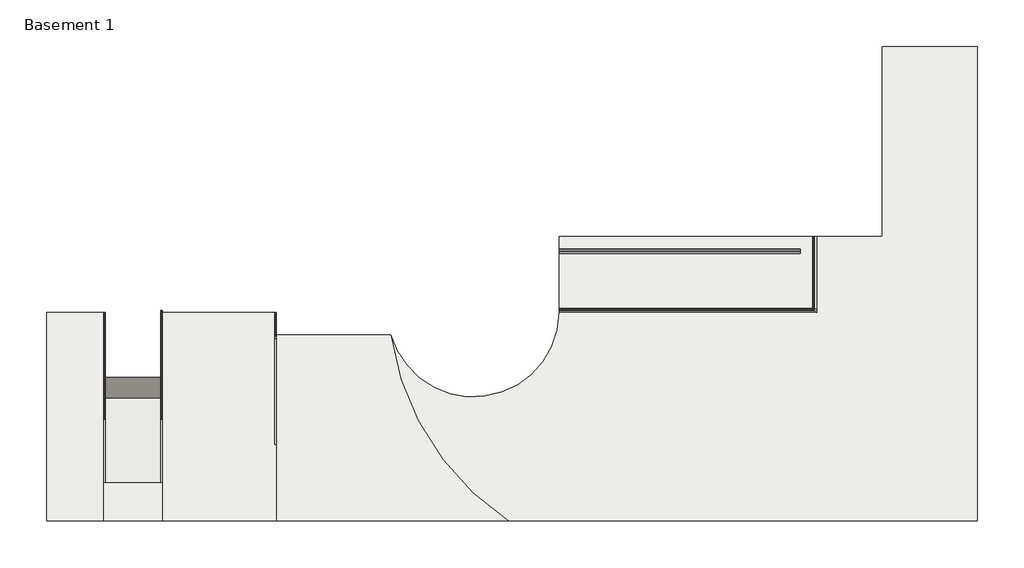
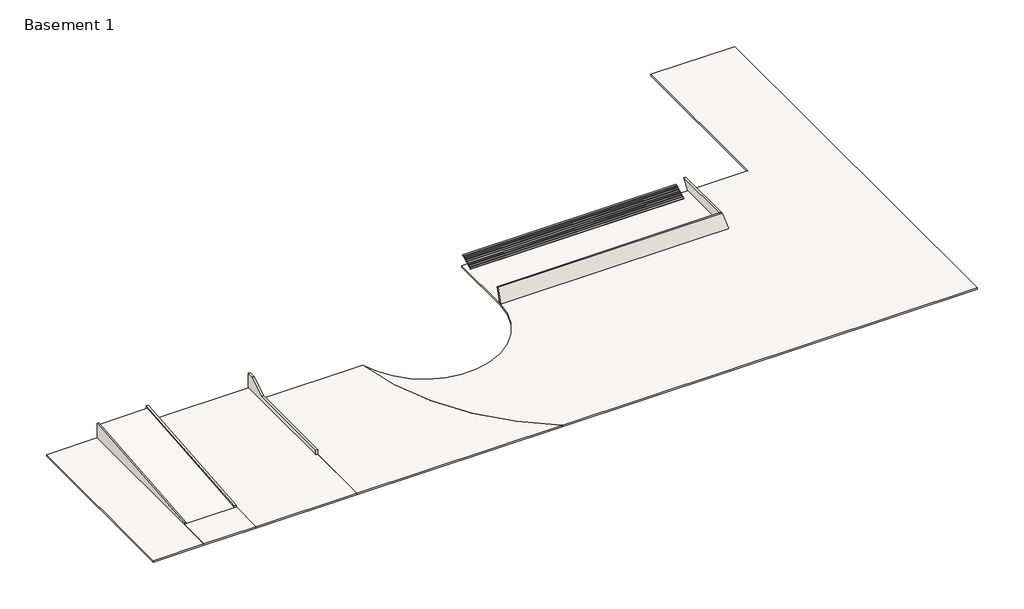
# One storey: 6 slabs, 5 walls, 1 stair flight.
"""IFC4 building model written with IfcOpenShell, lengths in millimetres."""

from ifc_helpers import new_model, si_unit, point, frame, frame_2d, origin, place, context, project, spatial, polyline, circle_curve, ellipse_curve, trimmed, segment, composite_curve, outline, extrude, faceted_brep, element, save
from ifc_brep_helpers import plane_surface, revolved_surface, advanced_brep

model = new_model("IFC4")

# Units and contexts
model_context = context("Model", 3, world=origin())
ifc_project = project(units=[si_unit("LENGTHUNIT", "METRE", prefix="MILLI")], contexts=[model_context])

# Site, building, storey
site = spatial("IfcSite", under=ifc_project)
building = spatial("IfcBuilding", under=site)
storey = spatial("IfcBuildingStorey", under=building, Name="Basement 1", Elevation=-2590.8)

# Slabs
placement = place(None, origin())
element("IfcSlab", 1, ObjectType="a_drive", at=placement, inside=storey, context=model_context, shape_type="SweptSolid", body=[
    extrude(outline(polyline([(19188.911889, -458.4117136), (-8130.1793721, -2896.8117136), (-8130.1793721, -2590.8), (19188.911889, -152.4), (19188.911889, -458.4117136)])), frame((-52722.4307976, 0.0, 0.0), z_axis=(1.0, 0.0, 0.0), x_axis=(0.0, 1.0, 0.0)), (0.0, 0.0, 1.0), 8839.2),
])
element("IfcSlab", 2, ObjectType="a_drive", at=placement, inside=storey, context=model_context, shape_type="SweptSolid", body=[
    extrude(outline(polyline([(-53027.2307976, -8130.1793721), (-43578.4307976, -8130.1793721), (-43578.4307976, -14339.088111), (-53027.2307976, -14339.088111), (-53027.2307976, -8130.1793721)])), frame((0.0, 0.0, -2895.6), z_axis=(0.0, 0.0, 1.0), x_axis=(1.0, 0.0, 0.0)), (0.0, 0.0, 1.0), 304.8),
])
element("IfcSlab", 3, ObjectType="a_site field", at=placement, inside=storey, context=model_context, shape_type="SweptSolid", body=[
    extrude(outline(composite_curve([segment(polyline([(20124.7692024, 31380.911889), (71940.7692024, 31380.911889), (71940.7692024, 61860.911889), (87180.7692024, 61860.911889), (87180.7692024, -14339.088111), (11898.6110424, -14339.088111)]), True, "CONTINUOUS"), segment(trimmed(circle_curve(frame_2d((35078.8556976, 21137.4265857)), 42378.1410317), [point((11898.6110424, -14339.088111))], [point((-6930.2202358, 15556.7118891))], False, "CARTESIAN"), True, "CONTINUOUS"), segment(trimmed(circle_curve(frame_2d((6325.7581451, 19397.6292514)), 13801.2176644), [point((-6930.2202358, 15556.7118891))], [point((20124.7692024, 19150.8442002))], True, "CARTESIAN"), True, "CONTINUOUS"), segment(polyline([(20124.7692024, 19150.8442002), (20124.7692024, 31380.911889)]), True, "CONTINUOUS")], self_intersect=False)), frame((0.0, 0.0, -2895.6), z_axis=(0.0, 0.0, 1.0), x_axis=(1.0, 0.0, 0.0)), (0.0, 0.0, 1.0), 304.8),
])
element("IfcSlab", 4, ObjectType="a_site field", at=placement, inside=storey, context=model_context, shape_type="SweptSolid", body=[
    extrude(outline(polyline([(-62171.2307976, 19188.911889), (-53027.2307976, 19188.911889), (-53027.2307976, -14339.088111), (-62171.2307976, -14339.088111), (-62171.2307976, 19188.911889)])), frame((0.0, 0.0, -2895.6), z_axis=(0.0, 0.0, 1.0), x_axis=(1.0, 0.0, 0.0)), (0.0, 0.0, 1.0), 304.8),
])
element("IfcSlab", 5, ObjectType="a_site field", at=placement, inside=storey, context=model_context, shape_type="SweptSolid", body=[
    extrude(outline(polyline([(-43578.4307976, 19188.911889), (-25290.4307976, 19188.911889), (-25290.4307976, -14339.088111), (-43578.4307976, -14339.088111), (-43578.4307976, 19188.911889)])), frame((0.0, 0.0, -2895.6), z_axis=(0.0, 0.0, 1.0), x_axis=(1.0, 0.0, 0.0)), (0.0, 0.0, 1.0), 304.8),
])
element("IfcSlab", 6, ObjectType="a_site paving", at=placement, inside=storey, context=model_context, shape_type="SweptSolid", body=[
    extrude(outline(composite_curve([segment(polyline([(-25290.4307976, 15556.711889), (-6930.2202358, 15556.711889)]), True, "CONTINUOUS"), segment(trimmed(circle_curve(frame_2d((35907.4785274, 21659.3058951)), 43270.1986236), [point((-6930.2202358, 15556.711889))], [point((11898.6110424, -14339.088111))], True, "CARTESIAN"), True, "CONTINUOUS"), segment(polyline([(11898.6110424, -14339.088111), (-25290.4307976, -14339.088111), (-25290.4307976, 15556.711889)]), True, "CONTINUOUS")], self_intersect=False)), frame((0.0, 0.0, -2895.6), z_axis=(0.0, 0.0, 1.0), x_axis=(1.0, 0.0, 0.0)), (0.0, 0.0, 1.0), 304.8),
])

# Stair flight
element("IfcStairFlight", 7, ObjectType="3/4\" Nosing", at=placement, inside=storey, context=model_context, shape_type="Brep", body=[
    faceted_brep([(58732.7692024, 28637.711889, -1507.0666667), (20124.7692024, 28637.711889, -1507.0666667), (20124.7692024, 28656.761889, -1676.4), (58732.7692024, 28656.761889, -1676.4), (58732.7692024, 28961.561889, -1507.0666667), (20124.7692024, 28961.561889, -1507.0666667), (20124.7692024, 28961.561889, -1579.7080571), (20124.7692024, 28787.5163918, -1676.4), (58732.7692024, 28787.5163918, -1676.4), (58732.7692024, 28961.561889, -1579.7080571), (20124.7692024, 28942.511889, -1337.7333333), (58732.7692024, 28942.511889, -1337.7333333), (58732.7692024, 29266.361889, -1337.7333333), (20124.7692024, 29266.361889, -1337.7333333), (20124.7692024, 29266.361889, -1410.3747238), (58732.7692024, 29266.361889, -1410.3747238), (20124.7692024, 29571.161889, -1241.0413904), (20124.7692024, 29875.961889, -1071.7080571), (20124.7692024, 30180.761889, -902.3747238), (20124.7692024, 30485.561889, -733.0413904), (20124.7692024, 30790.361889, -563.7080571), (20124.7692024, 31076.111889, -404.9580571), (58732.7692024, 31076.111889, -404.9580571), (58732.7692024, 30790.361889, -563.7080571), (58732.7692024, 30485.561889, -733.0413904), (58732.7692024, 30180.761889, -902.3747238), (58732.7692024, 29875.961889, -1071.7080571), (58732.7692024, 29571.161889, -1241.0413904), (20124.7692024, 29247.311889, -1168.4), (58732.7692024, 29247.311889, -1168.4), (58732.7692024, 29571.161889, -1168.4), (20124.7692024, 29571.161889, -1168.4), (20124.7692024, 29552.111889, -999.0666667), (58732.7692024, 29552.111889, -999.0666667), (58732.7692024, 29875.961889, -999.0666667), (20124.7692024, 29875.961889, -999.0666667), (20124.7692024, 29856.911889, -829.7333333), (58732.7692024, 29856.911889, -829.7333333), (58732.7692024, 30180.761889, -829.7333333), (20124.7692024, 30180.761889, -829.7333333), (20124.7692024, 30161.711889, -660.4), (58732.7692024, 30161.711889, -660.4), (58732.7692024, 30485.561889, -660.4), (20124.7692024, 30485.561889, -660.4), (20124.7692024, 30466.511889, -491.0666667), (58732.7692024, 30466.511889, -491.0666667), (58732.7692024, 30790.361889, -491.0666667), (20124.7692024, 30790.361889, -491.0666667), (20124.7692024, 30771.311889, -321.7333333), (58732.7692024, 30771.311889, -321.7333333), (58732.7692024, 31076.111889, -321.7333333), (20124.7692024, 31076.111889, -321.7333333)], [[[0, 1, 2, 3]], [[1, 0, 4, 5]], [[1, 5, 6, 7, 2]], [[4, 0, 3, 8, 9]], [[10, 11, 12, 13]], [[10, 13, 14, 6, 5]], [[12, 11, 4, 9, 15]], [[5, 4, 11, 10]], [[3, 2, 7, 8]], [[8, 7, 6, 14, 16, 17, 18, 19, 20, 21, 22, 23, 24, 25, 26, 27, 15, 9]], [[28, 29, 30, 31]], [[28, 31, 16, 14, 13]], [[30, 29, 12, 15, 27]], [[13, 12, 29, 28]], [[32, 33, 34, 35]], [[32, 35, 17, 16, 31]], [[34, 33, 30, 27, 26]], [[31, 30, 33, 32]], [[36, 37, 38, 39]], [[36, 39, 18, 17, 35]], [[38, 37, 34, 26, 25]], [[35, 34, 37, 36]], [[40, 41, 42, 43]], [[40, 43, 19, 18, 39]], [[42, 41, 38, 25, 24]], [[39, 38, 41, 40]], [[44, 45, 46, 47]], [[44, 47, 20, 19, 43]], [[46, 45, 42, 24, 23]], [[43, 42, 45, 44]], [[48, 49, 50, 51]], [[48, 51, 21, 20, 47]], [[50, 49, 46, 23, 22]], [[51, 50, 22, 21]], [[47, 46, 49, 48]]]),
])

# Walls
element("IfcWall", 8, ObjectType="Generic - 12\"", at=placement, inside=storey, context=model_context, shape_type="Brep", body=[
    faceted_brep([(-52722.4307976, -8130.1793721, -2590.8), (-52722.4307976, 19188.911889, -2590.8), (-52722.4307976, 19188.911889, 152.4), (-52722.4307976, 19188.911889, 153.6117136), (-52722.4307976, -8130.1793721, -2284.7882864), (-53027.2307976, -8130.1793721, -2590.8), (-53027.2307976, -8130.1793721, -2284.7882864), (-53027.2307976, 19188.911889, 153.6117136), (-53027.2307976, 19188.911889, -2590.8)], [[[0, 1, 2, 3, 4]], [[5, 6, 7, 8]], [[1, 0, 5, 8]], [[4, 3, 7, 6]], [[0, 4, 6, 5]], [[3, 2, 1, 8, 7]]]),
])
element("IfcWall", 9, ObjectType="Generic - 12\"", at=placement, inside=storey, context=model_context, shape_type="Brep", body=[
    faceted_brep([(-43578.4307976, -8130.1793721, -2590.8), (-43578.4307976, 19493.711889, -2590.8), (-43578.4307976, 19493.711889, -152.4), (-43578.4307976, 19493.711889, 152.4), (-43578.4307976, 19493.711889, 180.8170226), (-43578.4307976, -8130.1793721, -2284.7882864), (-43883.2307976, -8130.1793721, -2590.8), (-43883.2307976, -8130.1793721, -2284.7882864), (-43883.2307976, 19493.711889, 180.8170226), (-43883.2307976, 19493.711889, 152.4), (-43883.2307976, 19493.711889, -152.4), (-43883.2307976, 19493.711889, -2590.8)], [[[0, 1, 2, 3, 4, 5]], [[6, 7, 8, 9, 10, 11]], [[1, 0, 6, 11]], [[5, 4, 8, 7]], [[0, 5, 7, 6]], [[4, 3, 2, 1, 11, 10, 9, 8]]]),
])
element("IfcWall", 10, ObjectType="Generic - 12\"", at=placement, inside=storey, context=model_context, shape_type="SweptSolid", body=[
    extrude(outline(polyline([(-2034.1793721, -2590.8), (-2034.1793721, -1676.4), (14963.2558665, -1676.4), (17896.9558665, 152.4), (19188.911889, 152.4), (19188.911889, -2590.8), (-2034.1793721, -2590.8)])), frame((-25595.2307976, 0.0, 0.0), z_axis=(1.0, 0.0, 0.0), x_axis=(0.0, 1.0, 0.0)), (0.0, 0.0, 1.0), 304.8),
])
element("IfcWall", 11, ObjectType="a_panel enamel", at=placement, inside=storey, context=model_context, shape_type="AdvancedBrep", body=[
    advanced_brep(
    [(61430.5452923, 19499.0879789, -2590.8), (61430.5452923, 19183.5357991, -2590.8), (20123.8667318, 19183.5357991, -2590.8), (20124.7692024, 19341.311889, -2590.8), (20124.7692024, 19499.0879789, -2590.8), (61114.9931125, 19499.0879789, -2590.8), (60695.5070676, 20234.1262036, 152.4), (20124.7692024, 20234.1262036, 152.4), (60379.9548878, 20234.1262036, 152.4), (60695.5070676, 19918.5740238, 152.4), (20124.7692024, 19918.5740238, 152.4), (20124.7692024, 19341.311889, -2001.9716163)],
    [
        (0, 1),
        (1, 2),
        (2, 3, circle_curve(frame((6332.5692024, 19341.311889, -2590.8), z_axis=(0.0, 0.0, 1.0), x_axis=(0.0, -1.0, 0.0)), 13792.2)),
        (3, 4),
        (4, 5),
        (5, 0),
        (6, 0),
        (4, 7),
        (7, 8),
        (8, 6),
        (9, 6),
        (7, 10),
        (10, 9),
        (1, 9),
        (10, 11),
        (11, 2, ellipse_curve(frame((6332.5692024, 19341.311889, -2001.9716163), z_axis=(0.0, 0.9659258262890684, -0.25881904510252074), x_axis=(0.0, 0.25881904510252074, 0.9659258262890682)), 53288.9687254, 13792.2)),
        (11, 3),
    ],
    [
        plane_surface(frame((61272.7692024, 19183.5357991, -2590.8), z_axis=(0.0, 0.0, -1.0), x_axis=(-1.0, 0.0, 0.0))),
        plane_surface(frame((61272.7692024, 19499.0879789, -2590.8), z_axis=(0.0, 0.9659258262890684, -0.25881904510252074), x_axis=(-1.0, 0.0, 0.0))),
        plane_surface(frame((61272.7692024, 20234.1262036, 152.4), z_axis=(0.0, 0.0, 1.0), x_axis=(-1.0, 0.0, 0.0))),
        plane_surface(frame((61272.7692024, 19918.5740238, 152.4), z_axis=(0.0, -0.9659258262890684, 0.25881904510252074), x_axis=(-1.0, 0.0, 0.0))),
        plane_surface(frame((60695.5070676, 31228.511889, 152.4), z_axis=(0.9659258262890684, 0.0, 0.25881904510252074), x_axis=(0.0, -1.0, 0.0))),
        revolved_surface(polyline([(6332.5692024, 5549.111889, 49471.21953187431), (6332.5692024, 5549.111889, -53475.162764474306)]), (6332.5692024, 19341.311889, -2727.96), (0.0, 0.0, 1.0)),
        plane_surface(frame((20124.7692024, 39991.511889, -2727.96), z_axis=(-1.0, 0.0, 0.0), x_axis=(0.0, -1.0, 0.0))),
    ],
    [
        (0, [[1, 2, 3, 4, 5, 6]]),
        (1, [[7, -6, -5, 8, 9, 10]]),
        (2, [[11, -10, -9, 12, 13]]),
        (3, [[14, -13, 15, 16, -2]]),
        (4, [[-1, -7, -11, -14]]),
        (5, [[-16, 17, -3]]),
        (6, [[-15, -12, -8, -4, -17]]),
    ],
),
])
element("IfcWall", 12, ObjectType="a_panel enamel", at=placement, inside=storey, context=model_context, shape_type="Brep", body=[
    faceted_brep([(60379.9548878, 31380.911889, 152.4), (60543.2967155, 31380.911889, -457.2), (61114.9931125, 31380.911889, -2590.8), (61114.9931125, 31076.111889, -2590.8), (61114.9931125, 19499.0879789, -2590.8), (60379.9548878, 20234.1262036, 152.4), (61430.5452923, 31380.911889, -2590.8), (60695.5070676, 31380.911889, 152.4), (60695.5070676, 31076.111889, 152.4), (60695.5070676, 20234.1262036, 152.4), (61430.5452923, 19499.0879789, -2590.8), (61430.5452923, 31076.111889, -2590.8), (61272.7692024, 31380.911889, -2590.8)], [[[0, 1, 2, 3, 4, 5]], [[6, 7, 8, 9, 10, 11]], [[2, 12, 6, 11, 10, 4, 3]], [[7, 0, 5, 9, 8]], [[6, 12, 2, 1, 0, 7]], [[10, 9, 5, 4]]]),
])

save(model, "model.ifc")

# Revit data of these elements
# Project information
#   Project Issue Date = "Issue Date"
#   Project Status = "Project Status"
#   Client Name = "Owner"
#   Project Address = "Enter address here"
#   Project Name = "Project Name"
#   Project Number = "Project Number"
# Grids (mm)
#   "8": line (61272.769, 33542.122) -> (61272.769, 61407.715)
#   "7": line (52128.769, 33542.122) -> (52128.769, 61407.715)
#   "6": line (42984.769, 33542.122) -> (42984.769, 61407.715)
#   "5": line (33840.769, 33542.122) -> (33840.769, 61407.715)
#   "4": line (24696.769, 33542.122) -> (24696.769, 61407.715)
#   "3": line (15552.769, 33542.122) -> (15552.769, 61407.715)
#   "2": line (6408.769, 33542.122) -> (6408.769, 61407.715)
#   "1": line (-2735.231, 33542.122) -> (-2735.231, 61407.715)
#   "A": line (-6275.236, 57136.512) -> (64520.567, 57136.512)
#   "B": line (-6275.236, 47992.512) -> (64520.567, 47992.512)
#   "C": line (-6275.236, 38848.512) -> (64520.567, 38848.512)
# Type "a_drive"
#   Function = 0
#   Layers, outside or top first: 1' - 0" "a_drive" (function 0)
# Type "a_site field"
#   Function = 0
#   Layers, outside or top first: 1' - 0" "a_floor grass" (function 0)
# Type "a_site paving"
#   Function = 0
#   Layers, outside or top first: 1' - 0" "a_floor paving" (function 0)
# Type "Generic - 12\""
#   Assembly Code = "B2010"
#   Layers, outside or top first: 1' - 0" no material (function 1)
# Type "a_panel enamel"
#   Layers, outside or top first: 1' - 0" "a_panel enamel" (function 0)
# Elements 1, 2 (IfcSlab, "a_drive")
#   Height Offset From Level = 0' - 0"
#   Phase Created = New Construction
#   Materials on its faces: "a_drive"
# Elements 3, 4, 5 (IfcSlab, "a_site field")
#   Height Offset From Level = 0' - 0"
#   Phase Created = New Construction
#   Materials on its faces: "a_floor grass"
# Element 6 (IfcSlab, "a_site paving")
#   Height Offset From Level = 0' - 0"
#   Phase Created = New Construction
#   Materials on its faces: "a_floor paving"
# Element 7 (IfcStairFlight, "3/4\" Nosing")
#   Phase Created = New Construction
#   Materials on its faces: "Concrete, Cast-in-Place gray"
# Elements 8, 9, 10 (IfcWall, "Generic - 12\"")
#   Top Offset = 1' - 0"
#   Base Offset = 0' - 0"
#   wall height = 9' - 0"
#   Phase Created = New Construction
#   Base Constraint = Basement 1
#   Top Constraint = Site
#   Materials on its faces: "Default Wall"
# Elements 11, 12 (IfcWall, "a_panel enamel")
#   Top Offset = 1' - 0"
#   Base Offset = 0' - 0"
#   wall height = 9' - 0"
#   Phase Created = New Construction
#   Base Constraint = Basement 1
#   Top Constraint = Site
#   Materials on its faces: "a_panel enamel"
# Materials
#   "a_drive": class "Unassigned", colour RGB 0 0 0, transparency 0
#   "a_floor grass": class "Unassigned", colour RGB 104 134 53, transparency 0, Cost = 0
#   "a_floor paving": class "Unassigned", colour RGB 203 186 173, transparency 0, Cost = 0
#   "a_panel enamel": class "Unassigned", colour RGB 211 210 215, transparency 0, Comments = "Rendering appearance not upgraded "
#   "Concrete, Cast-in-Place gray": class "Concrete", colour RGB 192 192 192, transparency 0, Description = "Cast-in-place concrete", Cost = 0
#   "Default Wall": class "Miscellaneous", colour RGB 128 128 128, transparency 0, Cost = 0
